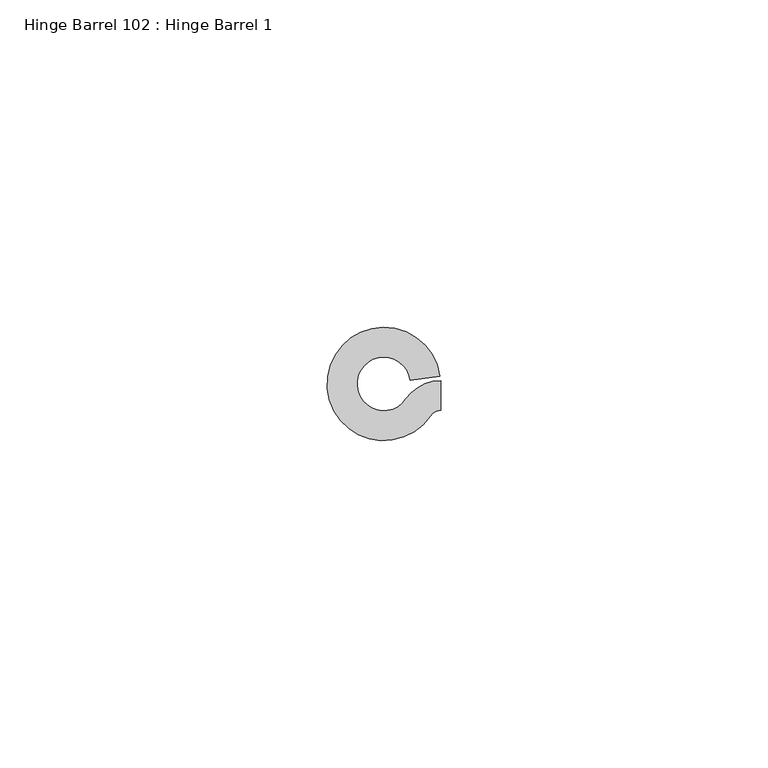
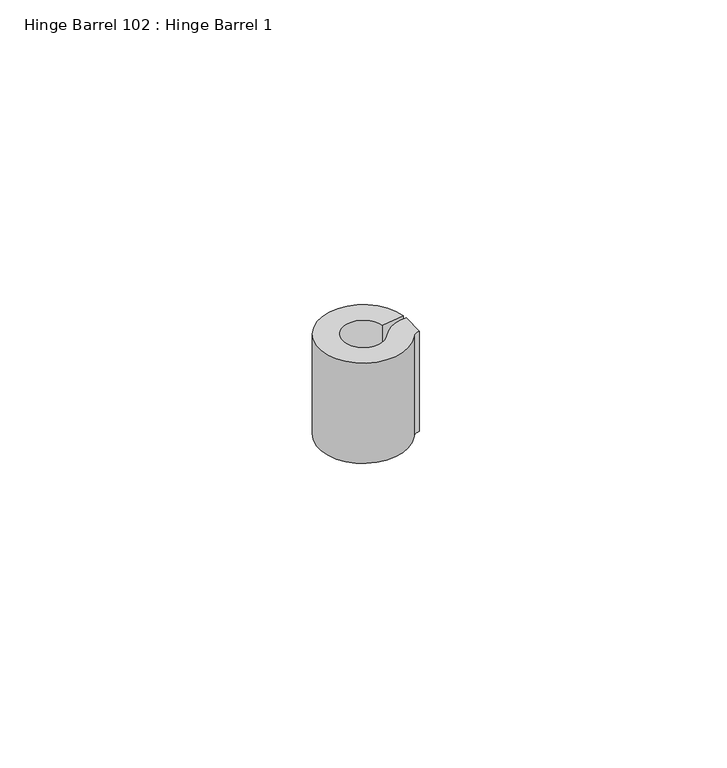
"""IFC4 building model written with IfcOpenShell, lengths in millimetres: proxy geometry, Hinge Barrel 102 : Hinge Barrel 1."""

from ifc_helpers import new_model, si_unit, point, frame, frame_2d, origin, place, context, project, spatial, polyline, circle_curve, trimmed, segment, composite_curve, outline, extrude, source, transform, mapped, element, save


def hinge_barrel_102_hinge_barrel_1_d5905ef5(model_context):
    return source(origin(), model_context, "Body", "SweptSolid", [
        extrude(outline(composite_curve([segment(trimmed(circle_curve(frame_2d((587327.8245257, -533990.5568067)), 6.4044851), [point((587322.5194669, -533986.9688017))], [point((587327.8245257, -533984.1523216))], False, "CARTESIAN"), True, "CONTINUOUS"), segment(polyline([(587327.8245257, -533984.1523216), (587327.8245257, -533988.7163841)]), True, "CONTINUOUS"), segment(trimmed(circle_curve(frame_2d((587327.8245257, -533990.5568067)), 1.8404226), [point((587327.8245257, -533988.7163841))], [point((587326.3000393, -533989.5257409))], True, "CARTESIAN"), True, "CONTINUOUS"), segment(trimmed(circle_curve(frame_2d((587319.1320739, -533984.6777841)), 8.6534625), [point((587326.3000393, -533989.5257409))], [point((587327.7022899, -533983.4803654))], False, "CARTESIAN"), True, "CONTINUOUS"), segment(polyline([(587327.7022899, -533983.4803654), (587323.1821338, -533984.1119153)]), True, "CONTINUOUS"), segment(trimmed(circle_curve(frame_2d((587319.1320739, -533984.6777841)), 4.0894), [point((587323.1821338, -533984.1119153))], [point((587322.5194669, -533986.9688017))], True, "CARTESIAN"), True, "CONTINUOUS")], self_intersect=False)), frame((0.0, 0.0, 2063.75), z_axis=(0.0, 0.0, 1.0), x_axis=(1.0, 0.0, 0.0)), (0.0, 0.0, 1.0), 20.8359375),
    ])


if __name__ == "__main__":
    model = new_model("IFC4")
    model_context = context("Model", 3, world=origin())
    ifc_project = project(units=[si_unit("LENGTHUNIT", "METRE", prefix="MILLI")], contexts=[model_context])
    site = spatial("IfcSite", under=ifc_project)
    building = spatial("IfcBuilding", under=site)
    placement = place(None, origin())
    hinge_barrel_102_hinge_barrel_1_shape = hinge_barrel_102_hinge_barrel_1_d5905ef5(model_context)
    element("IfcBuildingElementProxy", 1, Name="Hinge Barrel 102 : Hinge Barrel 1", ObjectType="Hinge Barrel 102 : Hinge Barrel 1", at=placement, inside=building, context=model_context, shape_type="MappedRepresentation", body=[
        mapped(hinge_barrel_102_hinge_barrel_1_shape, transform((0.0, 0.0, 0.0), x_axis=(1.0, 0.0, 0.0), y_axis=(0.0, 1.0, 0.0), z_axis=(0.0, 0.0, 1.0))),
    ])
    save(model, "model.ifc")

# Revit data of these elements
# Element 1 (IfcBuildingElementProxy, "Hinge Barrel 102 : Hinge Barrel 1")
#   Materials on its faces: "6\"X6\" WELD-ON STL BUTT HINGE"
# Materials
#   "6\"X6\" WELD-ON STL BUTT HINGE": class "Metal", colour RGB 189 187 185, transparency 0, Description = "Carbon steel", Cost = 0
